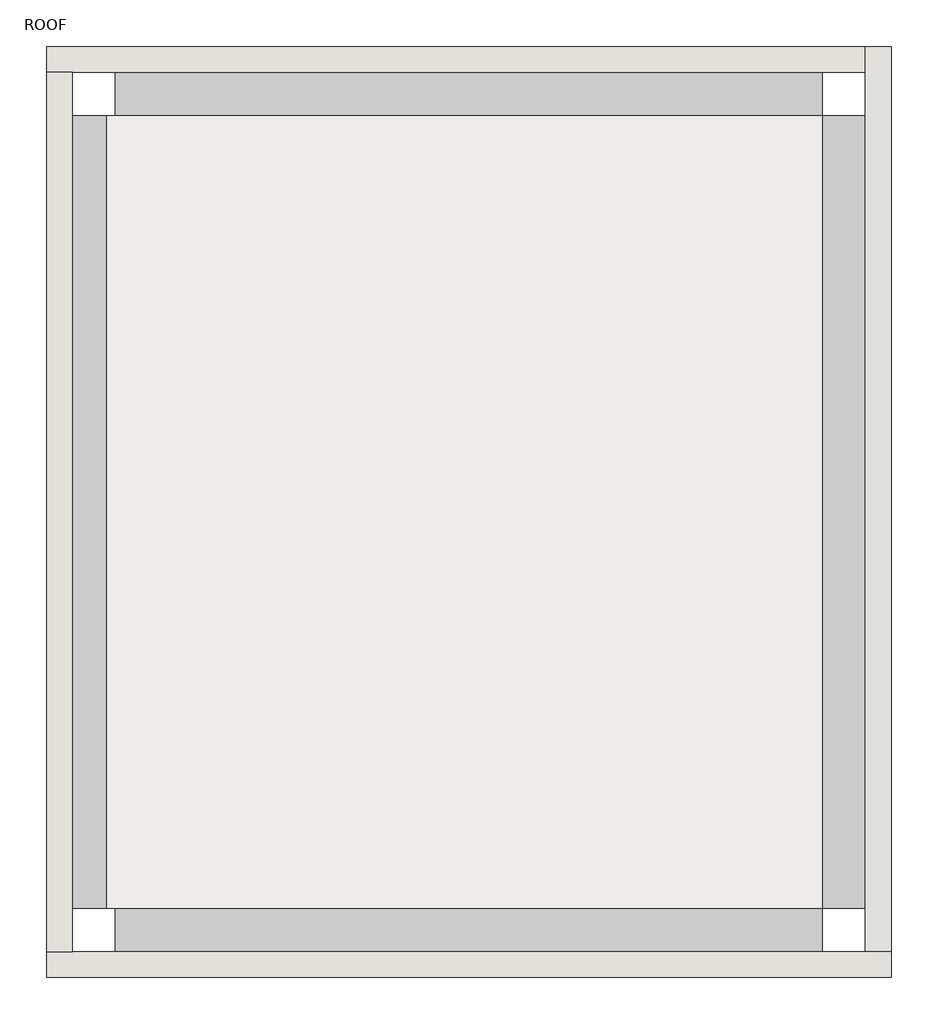
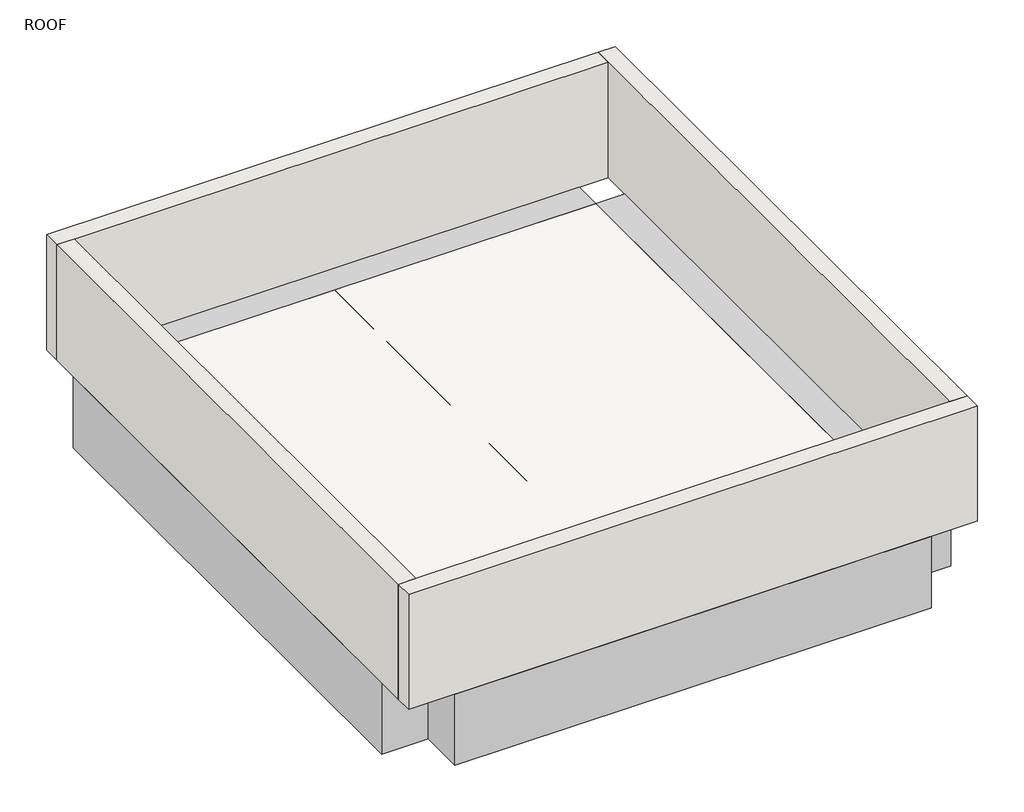
# One storey: 5 beams, 4 walls, 1 slab.
"""IFC4 building model written with IfcOpenShell, lengths in millimetres."""

from ifc_helpers import new_model, si_unit, frame, origin, place, context, project, spatial, polyline, outline, extrude, faceted_brep, element, save

model = new_model("IFC4")

# Units and contexts
model_context = context("Model", 3, world=origin())
ifc_project = project(units=[si_unit("LENGTHUNIT", "METRE", prefix="MILLI")], contexts=[model_context])

# Site, building, storey
site = spatial("IfcSite", under=ifc_project)
building = spatial("IfcBuilding", under=site)
storey = spatial("IfcBuildingStorey", under=building, Name="ROOF", Elevation=203400.0)

# Beams
placement = place(None, origin())
element("IfcBeam", 1, ObjectType="RC Beam_Rectangular : H_SB_ACB_B400xH650", at=placement, inside=storey, context=model_context, shape_type="Brep", body=[
    faceted_brep([(-1563.0, 4960.0208589, 203400.0), (-1563.0, 4560.0208589, 203400.0), (2537.0, 4560.0208589, 203400.0), (2537.0, 4960.0208589, 203400.0), (687.0, 4960.0208589, 203400.0), (287.0, 4960.0208589, 203400.0), (-1563.0, 4560.0208589, 202750.0), (2537.0, 4560.0208589, 202750.0), (-1563.0, 4960.0208589, 202750.0), (287.0, 4960.0208589, 202750.0), (687.0, 4960.0208589, 202750.0), (2537.0, 4960.0208589, 202750.0)], [[[0, 1, 2, 3, 4, 5]], [[1, 6, 7, 2]], [[6, 8, 9, 10, 11, 7]], [[8, 0, 5, 4, 3, 11, 10, 9]], [[8, 6, 1, 0]], [[3, 2, 7, 11]]]),
])
element("IfcBeam", 2, ObjectType="RC Beam_Rectangular : H_SB_ACB_B400xH650", at=placement, inside=storey, context=model_context, shape_type="SweptSolid", body=[
    extrude(outline(polyline([(-1963.0, 9560.0208589), (-1563.0, 9560.0208589), (-1563.0, 4960.0208589), (-1963.0, 4960.0208589), (-1963.0, 9560.0208589)])), frame((0.0, 0.0, 202750.0), z_axis=(0.0, 0.0, 1.0), x_axis=(1.0, 0.0, 0.0)), (0.0, 0.0, 1.0), 650.0),
])
element("IfcBeam", 3, ObjectType="RC Beam_Rectangular : H_SB_ACB_B400xH650", at=placement, inside=storey, context=model_context, shape_type="Brep", body=[
    faceted_brep([(2537.0, 9560.0208589, 203400.0), (2537.0, 9960.0208589, 203400.0), (-1563.0, 9960.0208589, 203400.0), (-1563.0, 9560.0208589, 203400.0), (287.0, 9560.0208589, 203400.0), (687.0, 9560.0208589, 203400.0), (-1563.0, 9560.0208589, 202750.0), (287.0, 9560.0208589, 202750.0), (687.0, 9560.0208589, 202750.0), (2537.0, 9560.0208589, 202750.0), (2537.0, 9960.0208589, 202750.0), (-1563.0, 9960.0208589, 202750.0)], [[[0, 1, 2, 3, 4, 5]], [[3, 6, 7, 8, 9, 0, 5, 4]], [[10, 9, 8, 7, 6, 11]], [[1, 10, 11, 2]], [[1, 0, 9, 10]], [[6, 3, 2, 11]]]),
])
element("IfcBeam", 4, ObjectType="RC Beam_Rectangular : H_SB_ACB_B400xH650", at=placement, inside=storey, context=model_context, shape_type="SweptSolid", body=[
    extrude(outline(polyline([(2537.0, 9560.0208589), (2937.0, 9560.0208589), (2937.0, 4960.0208589), (2537.0, 4960.0208589), (2537.0, 9560.0208589)])), frame((0.0, 0.0, 202750.0), z_axis=(0.0, 0.0, 1.0), x_axis=(1.0, 0.0, 0.0)), (0.0, 0.0, 1.0), 650.0),
])
element("IfcBeam", 5, ObjectType="RC Beam_Rectangular : H_SB_ACB_B400xH650", at=placement, inside=storey, context=model_context, shape_type="SweptSolid", body=[
    extrude(outline(polyline([(687.0, 4960.0208589), (287.0, 4960.0208589), (287.0, 9560.0208589), (687.0, 9560.0208589), (687.0, 4960.0208589)])), frame((0.0, 0.0, 202750.0), z_axis=(0.0, 0.0, 1.0), x_axis=(1.0, 0.0, 0.0)), (0.0, 0.0, 1.0), 650.0),
])

# Slab
element("IfcSlab", 6, ObjectType="H_FL_AMF_RC Slab_T150", at=placement, inside=storey, context=model_context, shape_type="SweptSolid", body=[
    extrude(outline(polyline([(2537.0, 9560.0208589), (2537.0, 4960.0208589), (-1613.0, 4960.0208589), (-1613.0, 9560.0208589), (2537.0, 9560.0208589)])), frame((0.0, 0.0, 203250.0), z_axis=(0.0, 0.0, 1.0), x_axis=(1.0, 0.0, 0.0)), (0.0, 0.0, 1.0), 150.0),
])

# Walls
element("IfcWall", 7, ObjectType="H_WA_AMW_RC Wall_T150 (No Finish)_PARAPET", at=placement, inside=storey, context=model_context, shape_type="Brep", body=[
    faceted_brep([(-1963.0, 4560.0208589, 203400.0), (2937.0, 4560.0208589, 203400.0), (2937.0, 4560.0208589, 204450.0), (-1963.0, 4560.0208589, 204450.0), (-1963.0, 4710.0208589, 203400.0), (-1963.0, 4710.0208589, 204450.0), (-1813.0, 4710.0208589, 204450.0), (2787.0, 4710.0208589, 204450.0), (2937.0, 4710.0208589, 204450.0), (2937.0, 4710.0208589, 203400.0), (2787.0, 4710.0208589, 203400.0), (-1813.0, 4710.0208589, 203400.0)], [[[0, 1, 2, 3]], [[4, 5, 6, 7, 8, 9, 10, 11]], [[0, 3, 5, 4]], [[1, 0, 4, 11, 10, 9]], [[3, 2, 8, 7, 6, 5]], [[2, 1, 9, 8]]]),
])
element("IfcWall", 8, ObjectType="H_WA_AMW_RC Wall_T150 (No Finish)_PARAPET", at=placement, inside=storey, context=model_context, shape_type="Brep", body=[
    faceted_brep([(2937.0, 4710.0208589, 203400.0), (2937.0, 9960.0208589, 203400.0), (2937.0, 9960.0208589, 204450.0), (2937.0, 4710.0208589, 204450.0), (2787.0, 4710.0208589, 203400.0), (2787.0, 4710.0208589, 204450.0), (2787.0, 9810.0208589, 204450.0), (2787.0, 9960.0208589, 204450.0), (2787.0, 9960.0208589, 203400.0), (2787.0, 9810.0208589, 203400.0)], [[[0, 1, 2, 3]], [[4, 5, 6, 7, 8, 9]], [[2, 1, 8, 7]], [[1, 0, 4, 9, 8]], [[3, 2, 7, 6, 5]], [[0, 3, 5, 4]]]),
])
element("IfcWall", 9, ObjectType="H_WA_AMW_RC Wall_T150 (No Finish)_PARAPET", at=placement, inside=storey, context=model_context, shape_type="Brep", body=[
    faceted_brep([(2787.0, 9960.0208589, 203400.0), (-1963.0, 9960.0208589, 203400.0), (-1963.0, 9960.0208589, 204450.0), (2787.0, 9960.0208589, 204450.0), (2787.0, 9810.0208589, 203400.0), (2787.0, 9810.0208589, 204450.0), (-1813.0, 9810.0208589, 204450.0), (-1963.0, 9810.0208589, 204450.0), (-1963.0, 9810.0208589, 203400.0), (-1813.0, 9810.0208589, 203400.0)], [[[0, 1, 2, 3]], [[4, 5, 6, 7, 8, 9]], [[1, 0, 4, 9, 8]], [[3, 2, 7, 6, 5]], [[0, 3, 5, 4]], [[2, 1, 8, 7]]]),
])
element("IfcWall", 10, ObjectType="H_WA_AMW_RC Wall_T150 (No Finish)_PARAPET", at=placement, inside=storey, context=model_context, shape_type="SweptSolid", body=[
    extrude(outline(polyline([(-1963.0, 4710.0208589), (-1963.0, 9810.0208589), (-1813.0, 9810.0208589), (-1813.0, 4710.0208589), (-1963.0, 4710.0208589)])), frame((0.0, 0.0, 203400.0), z_axis=(0.0, 0.0, 1.0), x_axis=(1.0, 0.0, 0.0)), (0.0, 0.0, 1.0), 1050.0),
])

save(model, "model.ifc")

# Revit data of these elements
# Type "RC Beam_Rectangular : H_SB_ACB_B400xH650"
#   중앙부 하부근 = ""
#   중앙부 상부근 = ""
#   중앙부 보조근 = ""
#   중앙부 늑근 = ""
#   외단부 하부근 = ""
#   외단부 상부근 = ""
#   외단부 보조근 = ""
#   외단부 늑근 = ""
#   부호 = "TG3"
#   내단부 하부근 = ""
#   내단부 상부근 = ""
#   내단부 보조근 = ""
#   내단부 늑근 = ""
#   ALL 하부근 = "3-D20"
#   ALL 상부근 = "3-D20"
#   ALL 보조근 = ""
#   ALL 늑근 = "2-D10 @120"
#   Width = 400.000 mm
#   Height = 650.000 mm
#   Length [instance default] = 1524.000 mm
#   b = 400.000 mm
#   h = 650.000 mm
#   hec_material3 [instance default] = none
#   hec_material2 [instance default] = none
#   hec_material1 [instance default] = none
#   Structural Material [instance default] = none
#   Assembly Code = ""
# Type "H_FL_AMF_RC Slab_T150"
#   Keynote = ""
#   Type Comments = ""
#   Description = ""
#   Function = 1
#   Layers, outside or top first: 150.000 mm no material (function 1)
# Type "H_WA_AMW_RC Wall_T150 (No Finish)_PARAPET"
#   Type Comments = ""
#   Layers, outside or top first: 0.000 mm no material (function 100); 0.000 mm no material (function 100); 150.000 mm no material (function 1); 0.000 mm no material (function 100); 0.000 mm no material (function 100); 0.000 mm no material (function 100)
# Elements 1, 2, 3, 4, 5 (IfcBeam, "RC Beam_Rectangular : H_SB_ACB_B400xH650")
#   hec_material3 = none
#   hec_material2 = none
#   hec_material1 = none
#   Structural Material = none
#   Phase Created = New Construction
# Element 6 (IfcSlab, "H_FL_AMF_RC Slab_T150")
#   Height Offset From Level = 0.000 mm
#   Phase Created = New Construction
#   Materials on its faces: "Default Floor"
# Elements 7, 9, 10 (IfcWall, "H_WA_AMW_RC Wall_T150 (No Finish)_PARAPET")
#   Top Offset = 0.000 mm
#   Base Offset = 0.000 mm
#   Unconnected Height = 1050.000 mm
#   wall height = 1050.000 mm
#   Phase Created = New Construction
#   Base Constraint = ROOF
#   Materials on its faces: "Default Wall"
# Element 8 (IfcWall, "H_WA_AMW_RC Wall_T150 (No Finish)_PARAPET")
#   Top Offset = 0.000 mm
#   Base Offset = 0.000 mm
#   Unconnected Height = 1050.000 mm
#   wall height = 1050.000 mm
#   Phase Created = New Construction
#   Base Constraint = ROOF
#   Top Constraint = PARAPET
#   Materials on its faces: "Default Wall"
# Materials
#   "Default Floor": class "Miscellaneous", colour RGB 80 80 80, transparency 0
#   "Default Wall": class "Miscellaneous", colour RGB 80 80 80, transparency 0
